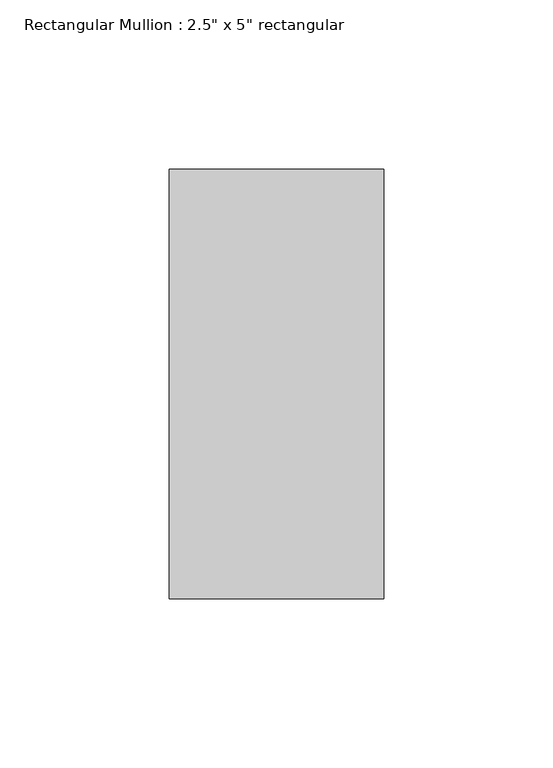
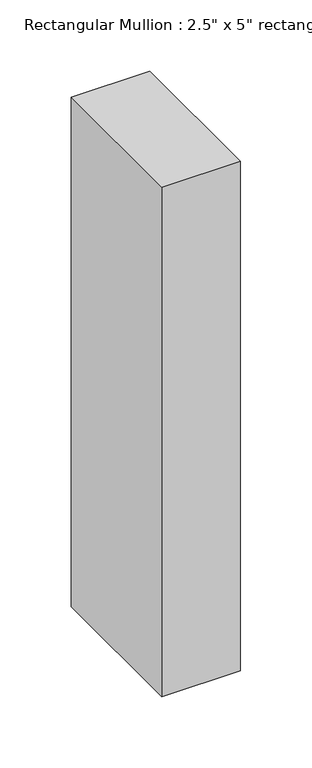
"""IFC4 building model written with IfcOpenShell, lengths in millimetres: member geometry."""

from ifc_helpers import new_model, si_unit, frame, origin, place, context, project, spatial, polyline, outline, extrude, source, transform, mapped, element, save


def member_59623374(model_context):
    return source(origin(), model_context, "Body", "SweptSolid", [
        extrude(outline(polyline([(31.75, 63.5), (31.75, -63.5), (-31.75, -63.5), (-31.75, 63.5), (31.75, 63.5)])), frame((0.0, 0.0, -435.6780939), z_axis=(0.0, 0.0, 1.0), x_axis=(1.0, 0.0, 0.0)), (0.0, 0.0, 1.0), 435.6780939),
    ])


if __name__ == "__main__":
    model = new_model("IFC4")
    model_context = context("Model", 3, world=origin())
    ifc_project = project(units=[si_unit("LENGTHUNIT", "METRE", prefix="MILLI")], contexts=[model_context])
    site = spatial("IfcSite", under=ifc_project)
    building = spatial("IfcBuilding", under=site)
    placement = place(None, origin())
    member_shape = member_59623374(model_context)
    element("IfcMember", 1, ObjectType="Rectangular Mullion : 2.5\" x 5\" rectangular", at=placement, inside=building, context=model_context, shape_type="MappedRepresentation", body=[
        mapped(member_shape, transform((0.0, 0.0, 0.0), x_axis=(1.0, 0.0, 0.0), y_axis=(0.0, 1.0, 0.0), z_axis=(0.0, 0.0, 1.0))),
    ])
    save(model, "model.ifc")

# Revit data of these elements
# Type "Rectangular Mullion : 2.5\" x 5\" rectangular"
#   built-in parameter 1007304 = 0.416667 (stored number, unit not read)
#   built-in parameter 1007301 = 0.104167 (stored number, unit not read)
#   built-in parameter 1007300 = 0.104167 (stored number, unit not read)
# Element 1 (IfcMember, "Rectangular Mullion : 2.5\" x 5\" rectangular")
#   Materials on its faces: "Metal - Aluminum 2"
# Materials
#   "Metal - Aluminum 2": class "Metal", colour RGB 189 187 185, transparency 0
